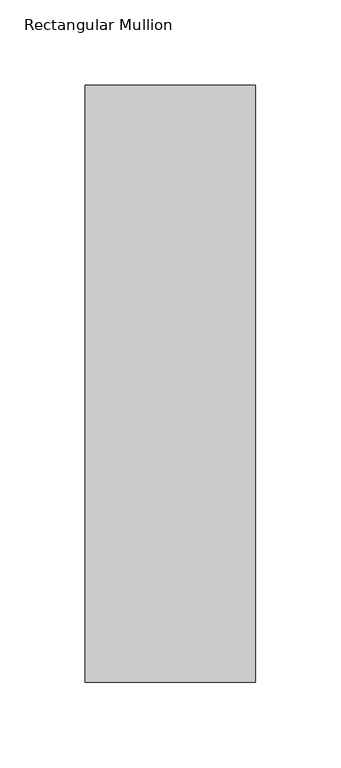
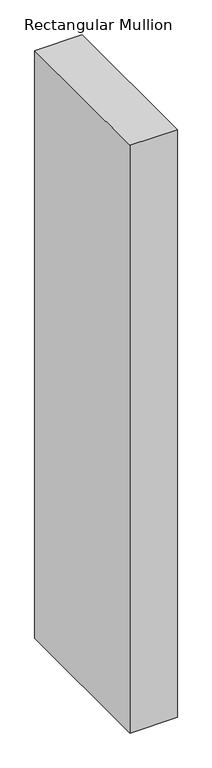
"""IFC4 building model written with IfcOpenShell, lengths in millimetres: member geometry, Rectangular Mullion : WWm-100x350-100mmOffset."""

import ifcopenshell
import ifcopenshell.guid

model = None  # the IFC model being written
_history = None  # IfcOwnerHistory: only IFC2X3 demands one
_inside = {}  # id of a spatial element -> (the spatial element, [elements in it])
_under = {}  # id of a project, library or spatial element -> (it, [spatial elements below it])
_declared = {}  # id of a project -> (the project, [libraries it declares])
_typed = {}  # id of a type object -> (the type object, [elements of that type])
_made_of = {}  # id of a material, layer set ... -> (it, [elements and type objects made of it])


def new_model(schema):
    """Start an empty IFC model of exactly this schema.

    Asked for "IFC4X3", IfcOpenShell would pick the latest addendum, in which some entities
    have other attributes; the version numbers below select the first issue.
    IFC2X3 requires an IfcOwnerHistory on every rooted entity: one is made here for all.
    """
    global model, _history
    if schema == "IFC4X3":
        model = ifcopenshell.file(schema_version=(4, 3, 0, 0))
    else:
        model = ifcopenshell.file(schema=schema)
    _inside.clear()
    _under.clear()
    _declared.clear()
    _typed.clear()
    _made_of.clear()
    _history = None
    if model.schema == "IFC2X3":
        org = make("IfcOrganization", Name="unknown")
        user = make(
            "IfcPersonAndOrganization",
            ThePerson=make("IfcPerson", FamilyName="unknown"),
            TheOrganization=org,
        )
        app = make(
            "IfcApplication",
            ApplicationDeveloper=org,
            Version="unknown",
            ApplicationFullName="unknown",
            ApplicationIdentifier="unknown",
        )
        _history = make(
            "IfcOwnerHistory",
            OwningUser=user,
            OwningApplication=app,
            ChangeAction="ADDED",
            CreationDate=0,
        )
    return model


def make(cls, **values):
    """One entity of the class cls with the attributes given. An attribute that is None is left unset."""
    return model.create_entity(
        cls, **{name: value for name, value in values.items() if value is not None}
    )


def rooted(cls, **values):
    """An entity with a GlobalId (a new one), such as an element, a storey or a relation."""
    return make(cls, GlobalId=ifcopenshell.guid.new(), OwnerHistory=_history, **values)


def si_unit(unit_type, name, prefix=None):
    """IfcSIUnit, for example si_unit("LENGTHUNIT", "METRE", prefix="MILLI")."""
    return make("IfcSIUnit", UnitType=unit_type, Prefix=prefix, Name=name)


def assignment(units):
    """IfcUnitAssignment: the units of a project."""
    return None if units is None else make("IfcUnitAssignment", Units=units)


def point(xyz):
    """IfcCartesianPoint."""
    return None if xyz is None else make("IfcCartesianPoint", Coordinates=xyz)


def direction(xyz):
    """IfcDirection."""
    return None if xyz is None else make("IfcDirection", DirectionRatios=xyz)


def frame(location, z_axis=None, x_axis=None):
    """IfcAxis2Placement3D, a coordinate frame: its origin and axes. An axis left out is left unset."""
    return make(
        "IfcAxis2Placement3D",
        Location=point(location),
        Axis=direction(z_axis),
        RefDirection=direction(x_axis),
    )


def origin():
    """The frame at (0, 0, 0) with its axes left unset."""
    return frame((0.0, 0.0, 0.0))


def place(relative_to, where):
    """IfcLocalPlacement: puts the frame where relative to a parent placement (None: the world)."""
    return make(
        "IfcLocalPlacement", PlacementRelTo=relative_to, RelativePlacement=where
    )


def context(
    kind, dimensions, precision=None, world=None, true_north=None, identifier=None
):
    """IfcGeometricRepresentationContext, for example the 3D "Model" context."""
    return make(
        "IfcGeometricRepresentationContext",
        ContextIdentifier=identifier,
        ContextType=kind,
        CoordinateSpaceDimension=dimensions,
        Precision=precision,
        WorldCoordinateSystem=world,
        TrueNorth=true_north,
    )


def project(units=None, contexts=None):
    """IfcProject with its units and contexts."""
    return rooted(
        "IfcProject",
        Name="project",
        RepresentationContexts=contexts,
        UnitsInContext=assignment(units),
    )


def spatial(cls, under=None, at=None, **own):
    """A site, building, storey or space (cls), placed at a placement, below another one or the project."""
    s = rooted(cls, ObjectPlacement=at, **own)
    if under is not None:
        _under.setdefault(under.id(), (under, []))[1].append(s)
    return s


def polyline(points):
    """IfcPolyline through the points."""
    return make("IfcPolyline", Points=[point(p) for p in points])


def outline(outer, holes=None, kind="AREA"):
    """IfcArbitraryClosedProfileDef: a profile drawn as a closed curve; with holes, ...WithVoids."""
    if holes is None:
        return make("IfcArbitraryClosedProfileDef", ProfileType=kind, OuterCurve=outer)
    return make(
        "IfcArbitraryProfileDefWithVoids",
        ProfileType=kind,
        OuterCurve=outer,
        InnerCurves=holes,
    )


def extrude(swept, where, along, depth):
    """IfcExtrudedAreaSolid: the profile swept, set in the frame where, extruded along a direction by depth."""
    return make(
        "IfcExtrudedAreaSolid",
        SweptArea=swept,
        Position=where,
        ExtrudedDirection=direction(along),
        Depth=depth,
    )


def shape(context_of_items, identifier, shape_type, items):
    """IfcShapeRepresentation: the items that make up one representation, for example the "Body"."""
    return make(
        "IfcShapeRepresentation",
        ContextOfItems=context_of_items,
        RepresentationIdentifier=identifier,
        RepresentationType=shape_type,
        Items=items,
    )


def source(mapping_origin, context_of_items, identifier, shape_type, items):
    """IfcRepresentationMap: a shape defined once, which mapped items show again and again."""
    return make(
        "IfcRepresentationMap",
        MappingOrigin=mapping_origin,
        MappedRepresentation=shape(context_of_items, identifier, shape_type, items),
    )


def transform(
    local_origin,
    x_axis=None,
    y_axis=None,
    z_axis=None,
    scale=None,
    scale2=None,
    scale3=None,
    uniform=True,
):
    """IfcCartesianTransformationOperator3D, or its non-uniform kind. x_axis, y_axis, z_axis: its Axis1, 2, 3."""
    if uniform:
        return make(
            "IfcCartesianTransformationOperator3D",
            Axis1=direction(x_axis),
            Axis2=direction(y_axis),
            LocalOrigin=point(local_origin),
            Scale=scale,
            Axis3=direction(z_axis),
        )
    return make(
        "IfcCartesianTransformationOperator3DnonUniform",
        Axis1=direction(x_axis),
        Axis2=direction(y_axis),
        LocalOrigin=point(local_origin),
        Scale=scale,
        Axis3=direction(z_axis),
        Scale2=scale2,
        Scale3=scale3,
    )


def mapped(mapping_source, mapping_target):
    """IfcMappedItem: shows the shape of a source again, moved by a transform."""
    return make(
        "IfcMappedItem", MappingSource=mapping_source, MappingTarget=mapping_target
    )


def made_of(thing, what):
    """Note that an element or type object is made of a material, layer set ...; save() writes the relation."""
    if what is not None:
        _made_of.setdefault(what.id(), (what, []))[1].append(thing)
    return thing


def element(
    cls,
    number,
    at=None,
    inside=None,
    cuts=None,
    type_object=None,
    material=None,
    context=None,
    identifier="Body",
    shape_type=None,
    held_by="IfcProductDefinitionShape",
    body=None,
    shapes=None,
    **own,
):
    """One element of the class cls, such as IfcWall. Its Tag is "e" and its number.

    at: its placement. inside: the storey or other place that contains it. cuts: it is an
    opening in that element (IfcRelVoidsElement). A single representation is given by context,
    identifier, shape_type and body (its items); several are given by shapes. held_by: the class
    of the entity that holds the representations. save() writes the other relations.
    """
    e = rooted(cls, Tag="e%d" % number, ObjectPlacement=at, **own)
    if body is not None:
        shapes = [shape(context, identifier, shape_type, body)]
    if shapes is not None:
        e.Representation = make(held_by, Representations=shapes)
    if inside is not None:
        _inside.setdefault(inside.id(), (inside, []))[1].append(e)
    if cuts is not None:
        rooted(
            "IfcRelVoidsElement", RelatingBuildingElement=cuts, RelatedOpeningElement=e
        )
    if type_object is not None:
        _typed.setdefault(type_object.id(), (type_object, []))[1].append(e)
    return made_of(e, material)


def aggregate(whole, parts):
    """IfcRelAggregates: a whole, such as a stair, and the parts it consists of."""
    return rooted("IfcRelAggregates", RelatingObject=whole, RelatedObjects=parts)


def save(model, path):
    """Write the relations noted so far, then the file.

    IfcRelAggregates (storeys below a building ...), IfcRelContainedInSpatialStructure (elements
    in a storey), IfcRelDefinesByType, IfcRelAssociatesMaterial and IfcRelDeclares: one each for
    every whole, place, type object, material and project.
    """
    for whole, parts in _under.values():
        aggregate(whole, parts)
    for where, things in _inside.values():
        rooted(
            "IfcRelContainedInSpatialStructure",
            RelatedElements=things,
            RelatingStructure=where,
        )
    for kind, things in _typed.values():
        rooted("IfcRelDefinesByType", RelatedObjects=things, RelatingType=kind)
    for what, things in _made_of.values():
        rooted("IfcRelAssociatesMaterial", RelatedObjects=things, RelatingMaterial=what)
    for by, libraries in _declared.values():
        rooted("IfcRelDeclares", RelatingContext=by, RelatedDefinitions=libraries)
    model.write(path)


def rectangular_mullion_891525b1(model_context):
    return source(origin(), model_context, "Body", "SweptSolid", [
        extrude(outline(polyline([(0.0, 175.0), (0.0, -175.0), (-100.0, -175.0), (-100.0, 175.0), (0.0, 175.0)])), frame((0.0, 0.0, -1315.6611397), z_axis=(0.0, 0.0, 1.0), x_axis=(1.0, 0.0, 0.0)), (0.0, 0.0, 1.0), 1315.6611397),
    ])


if __name__ == "__main__":
    model = new_model("IFC4")
    model_context = context("Model", 3, world=origin())
    ifc_project = project(units=[si_unit("LENGTHUNIT", "METRE", prefix="MILLI")], contexts=[model_context])
    site = spatial("IfcSite", under=ifc_project)
    building = spatial("IfcBuilding", under=site)
    placement = place(None, origin())
    rectangular_mullion_shape = rectangular_mullion_891525b1(model_context)
    element("IfcMember", 1, ObjectType="Rectangular Mullion : WWm-100x350-100mmOffset", at=placement, inside=building, context=model_context, shape_type="MappedRepresentation", body=[
        mapped(rectangular_mullion_shape, transform((0.0, 0.0, 0.0), x_axis=(1.0, 0.0, 0.0), y_axis=(0.0, 1.0, 0.0), z_axis=(0.0, 0.0, 1.0))),
    ])
    save(model, "model.ifc")

# Revit data of these elements
# Type "Rectangular Mullion : WWm-100x350-100mmOffset"
#   built-in parameter 1007304 = 1.14829 (stored number, unit not read)
#   built-in parameter 1007301 = 0.164042 (stored number, unit not read)
#   built-in parameter 1007300 = 0.164042 (stored number, unit not read)
# Element 1 (IfcMember, "Rectangular Mullion : WWm-100x350-100mmOffset")
#   Materials on its faces: "WW-EC-RGB-Mullion"
# Materials
#   "WW-EC-RGB-Mullion": class "Generic", colour RGB 255 255 255, transparency 0, Comments = "If region requests black mullions, switch asset color to RGB 25-25-25", Description = "Generic Color", Cost = 0
